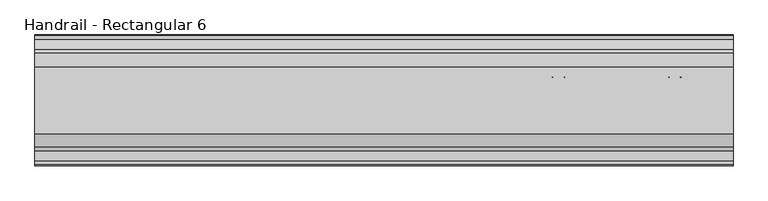
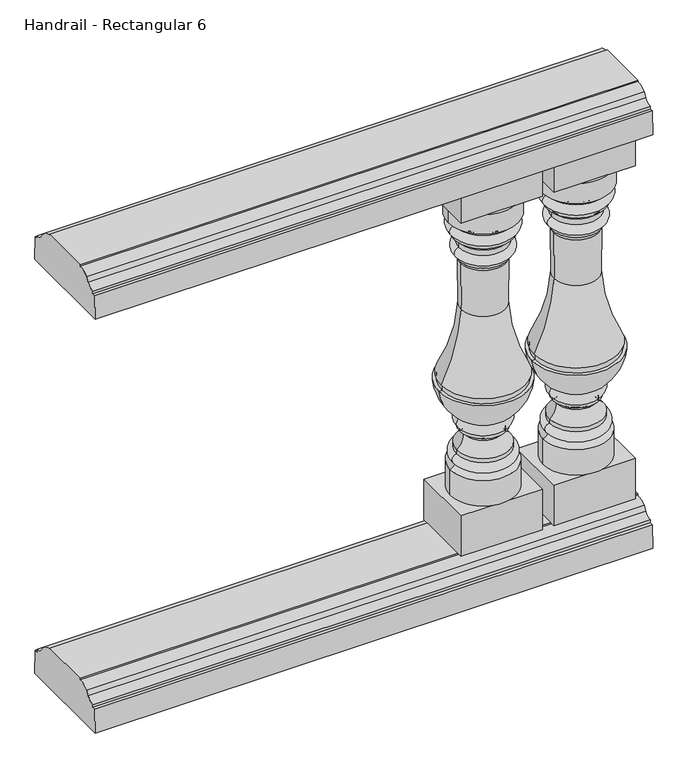
"""IFC4 building model written with IfcOpenShell, lengths in millimetres: railing geometry, Handrail - Rectangular 6."""

from ifc_helpers import new_model, si_unit, point, frame, frame_2d, origin, place, context, project, spatial, polyline, circle_curve, ellipse_curve, trimmed, segment, composite_curve, outline, extrude, source, transform, mapped, element, save
from ifc_brep_helpers import plane_surface, cylinder_surface, revolved_surface, advanced_brep


def handrail_rectangular_6_421e9862(model_context):
    return source(origin(), model_context, "Body", "SolidModel", [
        extrude(outline(composite_curve([segment(trimmed(circle_curve(frame_2d((-1771.1852268, 1054.89375)), 19.84375), [point((-1771.1852268, 1035.05))], [point((-1754.064785, 1044.8605607))], True, "CARTESIAN"), True, "CONTINUOUS"), segment(polyline([(-1754.064785, 1044.8605607), (-1747.604713, 1054.3201059)]), True, "CONTINUOUS"), segment(trimmed(circle_curve(frame_2d((-1723.5602268, 1027.90625)), 35.71875), [point((-1747.604713, 1054.3201059))], [point((-1723.5602268, 1063.625))], False, "CARTESIAN"), True, "CONTINUOUS"), segment(polyline([(-1723.5602268, 1063.625), (-1723.5602268, 1066.8), (-1607.6727268, 1066.8), (-1607.6727268, 1063.625)]), True, "CONTINUOUS"), segment(trimmed(circle_curve(frame_2d((-1607.6727268, 1027.90625)), 35.71875), [point((-1607.6727268, 1063.625))], [point((-1583.6282406, 1054.3201059))], False, "CARTESIAN"), True, "CONTINUOUS"), segment(polyline([(-1583.6282406, 1054.3201059), (-1577.1681686, 1044.8605607)]), True, "CONTINUOUS"), segment(trimmed(circle_curve(frame_2d((-1560.0477268, 1054.89375)), 19.84375), [point((-1577.1681686, 1044.8605607))], [point((-1560.0477268, 1035.05))], True, "CARTESIAN"), True, "CONTINUOUS"), segment(polyline([(-1560.0477268, 1035.05), (-1560.0477268, 1028.7), (-1552.9039768, 1028.7), (-1551.3164768, 974.725), (-1779.9164768, 974.725), (-1778.3289768, 1028.7), (-1771.1852268, 1028.7), (-1771.1852268, 1035.05)]), True, "CONTINUOUS")], self_intersect=False)), frame((18704.4521895, 0.0, 0.0), z_axis=(1.0, 0.0, 0.0), x_axis=(0.0, 1.0, 0.0)), (0.0, 0.0, 1.0), 1219.2),
        extrude(outline(composite_curve([segment(trimmed(circle_curve(frame_2d((-1771.1852268, 99.21875)), 19.84375), [point((-1771.1852268, 79.375))], [point((-1754.064785, 89.1855607))], True, "CARTESIAN"), True, "CONTINUOUS"), segment(polyline([(-1754.064785, 89.1855607), (-1747.604713, 98.6451059)]), True, "CONTINUOUS"), segment(trimmed(circle_curve(frame_2d((-1723.5602268, 72.23125)), 35.71875), [point((-1747.604713, 98.6451059))], [point((-1723.5602268, 107.95))], False, "CARTESIAN"), True, "CONTINUOUS"), segment(polyline([(-1723.5602268, 107.95), (-1723.5602268, 111.125), (-1607.6727268, 111.125), (-1607.6727268, 107.95)]), True, "CONTINUOUS"), segment(trimmed(circle_curve(frame_2d((-1607.6727268, 72.23125)), 35.71875), [point((-1607.6727268, 107.95))], [point((-1583.6282406, 98.6451059))], False, "CARTESIAN"), True, "CONTINUOUS"), segment(polyline([(-1583.6282406, 98.6451059), (-1577.1681686, 89.1855607)]), True, "CONTINUOUS"), segment(trimmed(circle_curve(frame_2d((-1560.0477268, 99.21875)), 19.84375), [point((-1577.1681686, 89.1855607))], [point((-1560.0477268, 79.375))], True, "CARTESIAN"), True, "CONTINUOUS"), segment(polyline([(-1560.0477268, 79.375), (-1560.0477268, 73.025), (-1552.9039768, 73.025), (-1551.3164768, 19.05), (-1779.9164768, 19.05), (-1778.3289768, 73.025), (-1771.1852268, 73.025), (-1771.1852268, 79.375)]), True, "CONTINUOUS")], self_intersect=False)), frame((18704.4521895, 0.0, 0.0), z_axis=(1.0, 0.0, 0.0), x_axis=(0.0, 1.0, 0.0)), (0.0, 0.0, 1.0), 1219.2),
        advanced_brep(
        [(19745.8521895, -1665.6164768, 881.0625), (19898.2521895, -1665.6164768, 881.0625), (19822.0521895, -1665.6164768, 881.0625), (19745.8521895, -1665.6164768, 835.3414358), (19898.2521895, -1665.6164768, 835.3414358), (19757.9812259, -1665.6164768, 824.1251909), (19886.1231531, -1665.6164768, 824.1251909), (19758.2264669, -1665.6164768, 801.0872354), (19885.8779121, -1665.6164768, 801.0872354), (19758.2264669, -1665.6164768, 792.9994382), (19885.8779121, -1665.6164768, 792.9994382), (19767.054986, -1665.6164768, 784.421477), (19877.049393, -1665.6164768, 784.421477), (19769.3912636, -1665.6164768, 770.116552), (19874.7131155, -1665.6164768, 770.116552), (19769.3912636, -1665.6164768, 748.0589375), (19874.7131155, -1665.6164768, 748.0589375), (19769.3912636, -1665.6164768, 739.775), (19874.7131155, -1665.6164768, 739.775), (19773.2635708, -1665.6164768, 732.0548389), (19870.8408083, -1665.6164768, 732.0548389), (19774.0730467, -1665.6164768, 625.8760562), (19870.0313324, -1665.6164768, 625.8760562), (19730.5137493, -1665.6164768, 465.93125), (19913.5906298, -1665.6164768, 465.93125), (19732.6156298, -1665.6164768, 465.93125), (19911.4887493, -1665.6164768, 465.93125), (19732.6156298, -1665.6164768, 453.23125), (19911.4887493, -1665.6164768, 453.23125), (19725.2146895, -1665.6164768, 453.23125), (19918.8896895, -1665.6164768, 453.23125), (19771.1407464, -1665.6164768, 375.8648455), (19872.9636327, -1665.6164768, 375.8648455), (19771.2821067, -1665.6164768, 352.5012686), (19872.8222724, -1665.6164768, 352.5012686), (19771.2821067, -1665.6164768, 345.021636), (19872.8222724, -1665.6164768, 345.021636), (19779.2341468, -1665.6164768, 336.1395712), (19864.8702323, -1665.6164768, 336.1395712), (19764.2656134, -1665.6164768, 304.3511281), (19879.8387657, -1665.6164768, 304.3511281), (19764.2656134, -1665.6164768, 295.0015923), (19879.8387657, -1665.6164768, 295.0015923), (19761.9267679, -1665.6164768, 273.4976463), (19882.1776112, -1665.6164768, 273.4976463), (19749.8419066, -1665.6164768, 263.7041906), (19894.2624725, -1665.6164768, 263.7041906), (19749.8419066, -1665.6164768, 204.7875), (19894.2624725, -1665.6164768, 204.7875), (19822.0521895, -1665.6164768, 204.7875)],
        [
            (0, 1, circle_curve(frame((19822.0521895, -1665.6164768, 881.0625), z_axis=(0.0, 0.0, 1.0), x_axis=(1.0, 0.0, 0.0)), 76.2)),
            (1, 2),
            (2, 0),
            (1, 0, circle_curve(frame((19822.0521895, -1665.6164768, 881.0625), z_axis=(0.0, 0.0, 1.0), x_axis=(1.0, 0.0, 0.0)), 76.2)),
            (3, 4, circle_curve(frame((19822.0521895, -1665.6164768, 835.3414358), z_axis=(0.0, 0.0, 1.0), x_axis=(1.0, 0.0, 0.0)), 76.2)),
            (4, 1),
            (0, 3),
            (4, 3, circle_curve(frame((19822.0521895, -1665.6164768, 835.3414358), z_axis=(0.0, 0.0, 1.0), x_axis=(1.0, 0.0, 0.0)), 76.2)),
            (5, 6, circle_curve(frame((19822.0521895, -1665.6164768, 824.1251909), z_axis=(0.0, 0.0, 1.0), x_axis=(1.0, 0.0, 0.0)), 64.0709636)),
            (6, 4, circle_curve(frame((19898.2657036, -1665.6164768, 823.1606434), z_axis=(0.0, 1.0, 0.0), x_axis=(-1.0, 0.0, 0.0)), 12.1807998)),
            (3, 5, circle_curve(frame((19745.8386755, -1665.6164768, 823.1606434), z_axis=(0.0, 1.0, 0.0), x_axis=(1.0, 0.0, 0.0)), 12.1807998)),
            (6, 5, circle_curve(frame((19822.0521895, -1665.6164768, 824.1251909), z_axis=(0.0, 0.0, 1.0), x_axis=(1.0, 0.0, 0.0)), 64.0709636)),
            (7, 8, circle_curve(frame((19822.0521895, -1665.6164768, 801.0872354), z_axis=(0.0, 0.0, 1.0), x_axis=(1.0, 0.0, 0.0)), 63.8257226)),
            (8, 6, circle_curve(frame((19883.7118198, -1665.6164768, 812.6305767), z_axis=(0.0, -1.0, 0.0), x_axis=(-1.0, 0.0, 0.0)), 11.7448152)),
            (5, 7, circle_curve(frame((19760.3925593, -1665.6164768, 812.6305767), z_axis=(0.0, -1.0, 0.0), x_axis=(1.0, 0.0, 0.0)), 11.7448152)),
            (8, 7, circle_curve(frame((19822.0521895, -1665.6164768, 801.0872354), z_axis=(0.0, 0.0, 1.0), x_axis=(1.0, 0.0, 0.0)), 63.8257226)),
            (9, 10, circle_curve(frame((19822.0521895, -1665.6164768, 792.9994382), z_axis=(0.0, 0.0, 1.0), x_axis=(1.0, 0.0, 0.0)), 63.8257226)),
            (10, 8),
            (7, 9),
            (10, 9, circle_curve(frame((19822.0521895, -1665.6164768, 792.9994382), z_axis=(0.0, 0.0, 1.0), x_axis=(1.0, 0.0, 0.0)), 63.8257226)),
            (11, 12, circle_curve(frame((19822.0521895, -1665.6164768, 784.421477), z_axis=(0.0, 0.0, 1.0), x_axis=(1.0, 0.0, 0.0)), 54.9972035)),
            (12, 10, circle_curve(frame((19890.2799215, -1665.6164768, 779.6366699), z_axis=(0.0, 1.0, 0.0), x_axis=(-1.0, 0.0, 0.0)), 14.06916)),
            (9, 11, circle_curve(frame((19753.8244576, -1665.6164768, 779.6366699), z_axis=(0.0, 1.0, 0.0), x_axis=(1.0, 0.0, 0.0)), 14.06916)),
            (12, 11, circle_curve(frame((19822.0521895, -1665.6164768, 784.421477), z_axis=(0.0, 0.0, 1.0), x_axis=(1.0, 0.0, 0.0)), 54.9972035)),
            (13, 14, circle_curve(frame((19822.0521895, -1665.6164768, 770.116552), z_axis=(0.0, 0.0, 1.0), x_axis=(1.0, 0.0, 0.0)), 52.660926)),
            (14, 12, circle_curve(frame((19903.672248, -1665.6164768, 772.7301948), z_axis=(0.0, 1.0, 0.0), x_axis=(-1.0, 0.0, 0.0)), 29.0768376)),
            (11, 13, circle_curve(frame((19740.4321311, -1665.6164768, 772.7301948), z_axis=(0.0, 1.0, 0.0), x_axis=(1.0, 0.0, 0.0)), 29.0768376)),
            (14, 13, circle_curve(frame((19822.0521895, -1665.6164768, 770.116552), z_axis=(0.0, 0.0, 1.0), x_axis=(1.0, 0.0, 0.0)), 52.660926)),
            (15, 16, circle_curve(frame((19822.0521895, -1665.6164768, 748.0589375), z_axis=(0.0, 0.0, 1.0), x_axis=(1.0, 0.0, 0.0)), 52.660926)),
            (16, 14, circle_curve(frame((19874.2588823, -1665.6164768, 759.0877448), z_axis=(0.0, -1.0, 0.0), x_axis=(-1.0, 0.0, 0.0)), 11.0381573)),
            (13, 15, circle_curve(frame((19769.8454968, -1665.6164768, 759.0877448), z_axis=(0.0, -1.0, 0.0), x_axis=(1.0, 0.0, 0.0)), 11.0381573)),
            (16, 15, circle_curve(frame((19822.0521895, -1665.6164768, 748.0589375), z_axis=(0.0, 0.0, 1.0), x_axis=(1.0, 0.0, 0.0)), 52.660926)),
            (17, 18, circle_curve(frame((19822.0521895, -1665.6164768, 739.775), z_axis=(0.0, 0.0, 1.0), x_axis=(1.0, 0.0, 0.0)), 52.660926)),
            (18, 16),
            (15, 17),
            (18, 17, circle_curve(frame((19822.0521895, -1665.6164768, 739.775), z_axis=(0.0, 0.0, 1.0), x_axis=(1.0, 0.0, 0.0)), 52.660926)),
            (19, 20, circle_curve(frame((19822.0521895, -1665.6164768, 732.0548389), z_axis=(0.0, 0.0, 1.0), x_axis=(1.0, 0.0, 0.0)), 48.7886187)),
            (20, 18, circle_curve(frame((19882.079759, -1665.6164768, 731.2487877), z_axis=(0.0, 1.0, 0.0), x_axis=(-1.0, 0.0, 0.0)), 11.2678184)),
            (17, 19, circle_curve(frame((19762.0246201, -1665.6164768, 731.2487877), z_axis=(0.0, 1.0, 0.0), x_axis=(1.0, 0.0, 0.0)), 11.2678184)),
            (20, 19, circle_curve(frame((19822.0521895, -1665.6164768, 732.0548389), z_axis=(0.0, 0.0, 1.0), x_axis=(1.0, 0.0, 0.0)), 48.7886187)),
            (21, 22, circle_curve(frame((19822.0521895, -1665.6164768, 625.8760562), z_axis=(0.0, 0.0, 1.0), x_axis=(1.0, 0.0, 0.0)), 47.9791428)),
            (22, 20, circle_curve(frame((20699.1718775, -1665.6164768, 672.6474087), z_axis=(0.0, 1.0, 0.0), x_axis=(-1.0, 0.0, 0.0)), 830.4586702)),
            (19, 21, circle_curve(frame((18944.9325016, -1665.6164768, 672.6474087), z_axis=(0.0, 1.0, 0.0), x_axis=(1.0, 0.0, 0.0)), 830.4586702)),
            (22, 21, circle_curve(frame((19822.0521895, -1665.6164768, 625.8760562), z_axis=(0.0, 0.0, 1.0), x_axis=(1.0, 0.0, 0.0)), 47.9791428)),
            (23, 24, circle_curve(frame((19822.0521895, -1665.6164768, 465.93125), z_axis=(0.0, 0.0, 1.0), x_axis=(1.0, 0.0, 0.0)), 91.5384403)),
            (24, 22, circle_curve(frame((20267.8631127, -1665.6164768, 648.3175235), z_axis=(0.0, 1.0, 0.0), x_axis=(-1.0, 0.0, 0.0)), 398.4642329)),
            (21, 23, circle_curve(frame((19376.2412664, -1665.6164768, 648.3175235), z_axis=(0.0, 1.0, 0.0), x_axis=(1.0, 0.0, 0.0)), 398.4642329)),
            (24, 23, circle_curve(frame((19822.0521895, -1665.6164768, 465.93125), z_axis=(0.0, 0.0, 1.0), x_axis=(1.0, 0.0, 0.0)), 91.5384403)),
            (25, 26, circle_curve(frame((19822.0521895, -1665.6164768, 465.93125), z_axis=(0.0, 0.0, 1.0), x_axis=(1.0, 0.0, 0.0)), 89.4365597)),
            (26, 24),
            (23, 25),
            (26, 25, circle_curve(frame((19822.0521895, -1665.6164768, 465.93125), z_axis=(0.0, 0.0, 1.0), x_axis=(1.0, 0.0, 0.0)), 89.4365597)),
            (27, 28, circle_curve(frame((19822.0521895, -1665.6164768, 453.23125), z_axis=(0.0, 0.0, 1.0), x_axis=(1.0, 0.0, 0.0)), 89.4365597)),
            (28, 26),
            (25, 27),
            (28, 27, circle_curve(frame((19822.0521895, -1665.6164768, 453.23125), z_axis=(0.0, 0.0, 1.0), x_axis=(1.0, 0.0, 0.0)), 89.4365597)),
            (29, 30, circle_curve(frame((19822.0521895, -1665.6164768, 453.23125), z_axis=(0.0, 0.0, 1.0), x_axis=(1.0, 0.0, 0.0)), 96.8375)),
            (30, 28),
            (27, 29),
            (30, 29, circle_curve(frame((19822.0521895, -1665.6164768, 453.23125), z_axis=(0.0, 0.0, 1.0), x_axis=(1.0, 0.0, 0.0)), 96.8375)),
            (31, 32, circle_curve(frame((19822.0521895, -1665.6164768, 375.8648455), z_axis=(0.0, 0.0, 1.0), x_axis=(1.0, 0.0, 0.0)), 50.9114432)),
            (32, 30, circle_curve(frame((19814.4105041, -1665.6164768, 462.9374706), z_axis=(0.0, -1.0, 0.0), x_axis=(-1.0, 0.0, 0.0)), 104.9290756)),
            (29, 31, circle_curve(frame((19829.6938749, -1665.6164768, 462.9374706), z_axis=(0.0, -1.0, 0.0), x_axis=(1.0, 0.0, 0.0)), 104.9290756)),
            (32, 31, circle_curve(frame((19822.0521895, -1665.6164768, 375.8648455), z_axis=(0.0, 0.0, 1.0), x_axis=(1.0, 0.0, 0.0)), 50.9114432)),
            (33, 34, circle_curve(frame((19822.0521895, -1665.6164768, 352.5012686), z_axis=(0.0, 0.0, 1.0), x_axis=(1.0, 0.0, 0.0)), 50.7700828)),
            (34, 32, circle_curve(frame((19867.5902787, -1665.6164768, 364.2151406), z_axis=(0.0, -1.0, 0.0), x_axis=(-1.0, 0.0, 0.0)), 12.8292072)),
            (31, 33, circle_curve(frame((19776.5141004, -1665.6164768, 364.2151406), z_axis=(0.0, -1.0, 0.0), x_axis=(1.0, 0.0, 0.0)), 12.8292072)),
            (34, 33, circle_curve(frame((19822.0521895, -1665.6164768, 352.5012686), z_axis=(0.0, 0.0, 1.0), x_axis=(1.0, 0.0, 0.0)), 50.7700828)),
            (35, 36, circle_curve(frame((19822.0521895, -1665.6164768, 345.021636), z_axis=(0.0, 0.0, 1.0), x_axis=(1.0, 0.0, 0.0)), 50.7700828)),
            (36, 34),
            (33, 35),
            (36, 35, circle_curve(frame((19822.0521895, -1665.6164768, 345.021636), z_axis=(0.0, 0.0, 1.0), x_axis=(1.0, 0.0, 0.0)), 50.7700828)),
            (37, 38, circle_curve(frame((19822.0521895, -1665.6164768, 336.1395712), z_axis=(0.0, 0.0, 1.0), x_axis=(1.0, 0.0, 0.0)), 42.8180427)),
            (38, 36, circle_curve(frame((19874.7676104, -1665.6164768, 335.27926), z_axis=(0.0, 1.0, 0.0), x_axis=(-1.0, 0.0, 0.0)), 9.9346983)),
            (35, 37, circle_curve(frame((19769.3367686, -1665.6164768, 335.27926), z_axis=(0.0, 1.0, 0.0), x_axis=(1.0, 0.0, 0.0)), 9.9346983)),
            (38, 37, circle_curve(frame((19822.0521895, -1665.6164768, 336.1395712), z_axis=(0.0, 0.0, 1.0), x_axis=(1.0, 0.0, 0.0)), 42.8180427)),
            (39, 40, circle_curve(frame((19822.0521895, -1665.6164768, 304.3511281), z_axis=(0.0, 0.0, 1.0), x_axis=(1.0, 0.0, 0.0)), 57.7865761)),
            (40, 38, circle_curve(frame((19899.6825509, -1665.6164768, 333.1135753), z_axis=(0.0, 1.0, 0.0), x_axis=(-1.0, 0.0, 0.0)), 34.9435857)),
            (37, 39, circle_curve(frame((19744.4218282, -1665.6164768, 333.1135753), z_axis=(0.0, 1.0, 0.0), x_axis=(1.0, 0.0, 0.0)), 34.9435857)),
            (40, 39, circle_curve(frame((19822.0521895, -1665.6164768, 304.3511281), z_axis=(0.0, 0.0, 1.0), x_axis=(1.0, 0.0, 0.0)), 57.7865761)),
            (41, 42, circle_curve(frame((19822.0521895, -1665.6164768, 295.0015923), z_axis=(0.0, 0.0, 1.0), x_axis=(1.0, 0.0, 0.0)), 57.7865761)),
            (42, 40),
            (39, 41),
            (42, 41, circle_curve(frame((19822.0521895, -1665.6164768, 295.0015923), z_axis=(0.0, 0.0, 1.0), x_axis=(1.0, 0.0, 0.0)), 57.7865761)),
            (43, 44, circle_curve(frame((19822.0521895, -1665.6164768, 273.4976463), z_axis=(0.0, 0.0, 1.0), x_axis=(1.0, 0.0, 0.0)), 60.1254216)),
            (44, 42, circle_curve(frame((19879.2247827, -1665.6164768, 284.0556497), z_axis=(0.0, -1.0, 0.0), x_axis=(-1.0, 0.0, 0.0)), 10.9631488)),
            (41, 43, circle_curve(frame((19764.8795963, -1665.6164768, 284.0556497), z_axis=(0.0, -1.0, 0.0), x_axis=(1.0, 0.0, 0.0)), 10.9631488)),
            (44, 43, circle_curve(frame((19822.0521895, -1665.6164768, 273.4976463), z_axis=(0.0, 0.0, 1.0), x_axis=(1.0, 0.0, 0.0)), 60.1254216)),
            (45, 46, circle_curve(frame((19822.0521895, -1665.6164768, 263.7041906), z_axis=(0.0, 0.0, 1.0), x_axis=(1.0, 0.0, 0.0)), 72.210283)),
            (46, 44, circle_curve(frame((19900.3933754, -1665.6164768, 283.622485), z_axis=(0.0, 1.0, 0.0), x_axis=(-1.0, 0.0, 0.0)), 20.8404996)),
            (43, 45, circle_curve(frame((19743.7110037, -1665.6164768, 283.622485), z_axis=(0.0, 1.0, 0.0), x_axis=(1.0, 0.0, 0.0)), 20.8404996)),
            (46, 45, circle_curve(frame((19822.0521895, -1665.6164768, 263.7041906), z_axis=(0.0, 0.0, 1.0), x_axis=(1.0, 0.0, 0.0)), 72.210283)),
            (47, 48, circle_curve(frame((19822.0521895, -1665.6164768, 204.7875), z_axis=(0.0, 0.0, 1.0), x_axis=(1.0, 0.0, 0.0)), 72.210283)),
            (48, 46),
            (45, 47),
            (48, 47, circle_curve(frame((19822.0521895, -1665.6164768, 204.7875), z_axis=(0.0, 0.0, 1.0), x_axis=(1.0, 0.0, 0.0)), 72.210283)),
            (49, 48),
            (47, 49),
        ],
        [
            plane_surface(frame((19822.0521895, -1665.6164768, 881.0625), z_axis=(0.0, 0.0, 1.0), x_axis=(1.0, 0.0, 0.0))),
            cylinder_surface(frame((19822.0521895, -1665.6164768, 833.4375), z_axis=(0.0, 0.0, -1.0), x_axis=(1.0, 0.0, 0.0)), 76.2),
            revolved_surface(trimmed(ellipse_curve(frame((19898.2657036, -1665.6164768, 823.1606434), z_axis=(0.0, -1.0, 0.0), x_axis=(-1.0, 0.0, 0.0)), 12.1807998, 12.1807998), [point((19898.2521895, -1665.6164768, 835.3414358))], [point((19886.1231531, -1665.6164768, 824.1251909))], True, "CARTESIAN"), (19822.0521895, -1665.6164768, 833.4375), (0.0, 0.0, -1.0)),
            revolved_surface(trimmed(ellipse_curve(frame((19883.7118198, -1665.6164768, 812.6305767), z_axis=(0.0, 1.0, 0.0), x_axis=(-1.0, 0.0, 0.0)), 11.7448152, 11.7448152), [point((19886.1231531, -1665.6164768, 824.1251909))], [point((19885.8779121, -1665.6164768, 801.0872354))], True, "CARTESIAN"), (19822.0521895, -1665.6164768, 833.4375), (0.0, 0.0, -1.0)),
            cylinder_surface(frame((19822.0521895, -1665.6164768, 833.4375), z_axis=(0.0, 0.0, -1.0), x_axis=(1.0, 0.0, 0.0)), 63.8257226),
            revolved_surface(trimmed(ellipse_curve(frame((19890.2799215, -1665.6164768, 779.6366699), z_axis=(0.0, -1.0, 0.0), x_axis=(-1.0, 0.0, 0.0)), 14.06916, 14.06916), [point((19885.8779121, -1665.6164768, 792.9994382))], [point((19877.049393, -1665.6164768, 784.421477))], True, "CARTESIAN"), (19822.0521895, -1665.6164768, 833.4375), (0.0, 0.0, -1.0)),
            revolved_surface(trimmed(ellipse_curve(frame((19903.672248, -1665.6164768, 772.7301948), z_axis=(0.0, -1.0, 0.0), x_axis=(-1.0, 0.0, 0.0)), 29.0768376, 29.0768376), [point((19877.049393, -1665.6164768, 784.421477))], [point((19874.7131155, -1665.6164768, 770.116552))], True, "CARTESIAN"), (19822.0521895, -1665.6164768, 833.4375), (0.0, 0.0, -1.0)),
            revolved_surface(trimmed(ellipse_curve(frame((19874.2588823, -1665.6164768, 759.0877448), z_axis=(0.0, 1.0, 0.0), x_axis=(-1.0, 0.0, 0.0)), 11.0381573, 11.0381573), [point((19874.7131155, -1665.6164768, 770.116552))], [point((19874.7131155, -1665.6164768, 748.0589375))], True, "CARTESIAN"), (19822.0521895, -1665.6164768, 833.4375), (0.0, 0.0, -1.0)),
            cylinder_surface(frame((19822.0521895, -1665.6164768, 833.4375), z_axis=(0.0, 0.0, -1.0), x_axis=(1.0, 0.0, 0.0)), 52.660926),
            revolved_surface(trimmed(ellipse_curve(frame((19882.079759, -1665.6164768, 731.2487877), z_axis=(0.0, -1.0, 0.0), x_axis=(-1.0, 0.0, 0.0)), 11.2678184, 11.2678184), [point((19874.7131155, -1665.6164768, 739.775))], [point((19870.8408083, -1665.6164768, 732.0548389))], True, "CARTESIAN"), (19822.0521895, -1665.6164768, 833.4375), (0.0, 0.0, -1.0)),
            revolved_surface(trimmed(ellipse_curve(frame((20699.1718775, -1665.6164768, 672.6474087), z_axis=(0.0, -1.0, 0.0), x_axis=(-1.0, 0.0, 0.0)), 830.4586702, 830.4586702), [point((19870.8408083, -1665.6164768, 732.0548389))], [point((19870.0313324, -1665.6164768, 625.8760562))], True, "CARTESIAN"), (19822.0521895, -1665.6164768, 833.4375), (0.0, 0.0, -1.0)),
            revolved_surface(trimmed(ellipse_curve(frame((20267.8631127, -1665.6164768, 648.3175235), z_axis=(0.0, -1.0, 0.0), x_axis=(-1.0, 0.0, 0.0)), 398.4642329, 398.4642329), [point((19870.0313324, -1665.6164768, 625.8760562))], [point((19913.5906298, -1665.6164768, 465.93125))], True, "CARTESIAN"), (19822.0521895, -1665.6164768, 833.4375), (0.0, 0.0, -1.0)),
            plane_surface(frame((19822.0521895, -1665.6164768, 465.93125), z_axis=(0.0, 0.0, -1.0), x_axis=(1.0, 0.0, 0.0))),
            cylinder_surface(frame((19822.0521895, -1665.6164768, 833.4375), z_axis=(0.0, 0.0, -1.0), x_axis=(1.0, 0.0, 0.0)), 89.4365597),
            plane_surface(frame((19822.0521895, -1665.6164768, 453.23125), z_axis=(0.0, 0.0, 1.0), x_axis=(1.0, 0.0, 0.0))),
            revolved_surface(trimmed(ellipse_curve(frame((19814.4105041, -1665.6164768, 462.9374706), z_axis=(0.0, 1.0, 0.0), x_axis=(-1.0, 0.0, 0.0)), 104.9290756, 104.9290756), [point((19918.8896895, -1665.6164768, 453.23125))], [point((19872.9636327, -1665.6164768, 375.8648455))], True, "CARTESIAN"), (19822.0521895, -1665.6164768, 833.4375), (0.0, 0.0, -1.0)),
            revolved_surface(trimmed(ellipse_curve(frame((19867.5902787, -1665.6164768, 364.2151406), z_axis=(0.0, 1.0, 0.0), x_axis=(-1.0, 0.0, 0.0)), 12.8292072, 12.8292072), [point((19872.9636327, -1665.6164768, 375.8648455))], [point((19872.8222724, -1665.6164768, 352.5012686))], True, "CARTESIAN"), (19822.0521895, -1665.6164768, 833.4375), (0.0, 0.0, -1.0)),
            cylinder_surface(frame((19822.0521895, -1665.6164768, 833.4375), z_axis=(0.0, 0.0, -1.0), x_axis=(1.0, 0.0, 0.0)), 50.7700828),
            revolved_surface(trimmed(ellipse_curve(frame((19874.7676104, -1665.6164768, 335.27926), z_axis=(0.0, -1.0, 0.0), x_axis=(-1.0, 0.0, 0.0)), 9.9346983, 9.9346983), [point((19872.8222724, -1665.6164768, 345.021636))], [point((19864.8702323, -1665.6164768, 336.1395712))], True, "CARTESIAN"), (19822.0521895, -1665.6164768, 833.4375), (0.0, 0.0, -1.0)),
            revolved_surface(trimmed(ellipse_curve(frame((19899.6825509, -1665.6164768, 333.1135753), z_axis=(0.0, -1.0, 0.0), x_axis=(-1.0, 0.0, 0.0)), 34.9435857, 34.9435857), [point((19864.8702323, -1665.6164768, 336.1395712))], [point((19879.8387657, -1665.6164768, 304.3511281))], True, "CARTESIAN"), (19822.0521895, -1665.6164768, 833.4375), (0.0, 0.0, -1.0)),
            cylinder_surface(frame((19822.0521895, -1665.6164768, 833.4375), z_axis=(0.0, 0.0, -1.0), x_axis=(1.0, 0.0, 0.0)), 57.7865761),
            revolved_surface(trimmed(ellipse_curve(frame((19879.2247827, -1665.6164768, 284.0556497), z_axis=(0.0, 1.0, 0.0), x_axis=(-1.0, 0.0, 0.0)), 10.9631488, 10.9631488), [point((19879.8387657, -1665.6164768, 295.0015923))], [point((19882.1776112, -1665.6164768, 273.4976463))], True, "CARTESIAN"), (19822.0521895, -1665.6164768, 833.4375), (0.0, 0.0, -1.0)),
            revolved_surface(trimmed(ellipse_curve(frame((19900.3933754, -1665.6164768, 283.622485), z_axis=(0.0, -1.0, 0.0), x_axis=(-1.0, 0.0, 0.0)), 20.8404996, 20.8404996), [point((19882.1776112, -1665.6164768, 273.4976463))], [point((19894.2624725, -1665.6164768, 263.7041906))], True, "CARTESIAN"), (19822.0521895, -1665.6164768, 833.4375), (0.0, 0.0, -1.0)),
            cylinder_surface(frame((19822.0521895, -1665.6164768, 833.4375), z_axis=(0.0, 0.0, -1.0), x_axis=(1.0, 0.0, 0.0)), 72.210283),
            plane_surface(frame((19822.0521895, -1665.6164768, 204.7875), z_axis=(0.0, 0.0, -1.0), x_axis=(1.0, 0.0, 0.0))),
        ],
        [
            (0, [[1, 2, 3]]),
            (0, [[4, -3, -2]]),
            (1, [[5, 6, -1, 7]]),
            (1, [[8, -7, -4, -6]]),
            (2, [[9, 10, -5, 11]]),
            (2, [[12, -11, -8, -10]]),
            (3, [[13, 14, -9, 15]]),
            (3, [[16, -15, -12, -14]]),
            (4, [[17, 18, -13, 19]]),
            (4, [[20, -19, -16, -18]]),
            (5, [[21, 22, -17, 23]]),
            (5, [[24, -23, -20, -22]]),
            (6, [[25, 26, -21, 27]]),
            (6, [[28, -27, -24, -26]]),
            (7, [[29, 30, -25, 31]]),
            (7, [[32, -31, -28, -30]]),
            (8, [[33, 34, -29, 35]]),
            (8, [[36, -35, -32, -34]]),
            (9, [[37, 38, -33, 39]]),
            (9, [[40, -39, -36, -38]]),
            (10, [[41, 42, -37, 43]]),
            (10, [[44, -43, -40, -42]]),
            (11, [[45, 46, -41, 47]]),
            (11, [[48, -47, -44, -46]]),
            (12, [[49, 50, -45, 51]]),
            (12, [[52, -51, -48, -50]]),
            (13, [[53, 54, -49, 55]]),
            (13, [[56, -55, -52, -54]]),
            (14, [[57, 58, -53, 59]]),
            (14, [[60, -59, -56, -58]]),
            (15, [[61, 62, -57, 63]]),
            (15, [[64, -63, -60, -62]]),
            (16, [[65, 66, -61, 67]]),
            (16, [[68, -67, -64, -66]]),
            (17, [[69, 70, -65, 71]]),
            (17, [[72, -71, -68, -70]]),
            (18, [[73, 74, -69, 75]]),
            (18, [[76, -75, -72, -74]]),
            (19, [[77, 78, -73, 79]]),
            (19, [[80, -79, -76, -78]]),
            (20, [[81, 82, -77, 83]]),
            (20, [[84, -83, -80, -82]]),
            (21, [[85, 86, -81, 87]]),
            (21, [[88, -87, -84, -86]]),
            (22, [[89, 90, -85, 91]]),
            (22, [[92, -91, -88, -90]]),
            (23, [[93, 94, -89, 95]]),
            (23, [[96, -95, -92, -94]]),
            (24, [[97, -93, 98]]),
            (24, [[-98, -96, -97]]),
        ],
    ),
        extrude(outline(polyline([(19733.1521895, -1735.4664768), (19733.1521895, -1595.7664768), (19910.9521895, -1595.7664768), (19910.9521895, -1735.4664768), (19733.1521895, -1735.4664768)])), frame((0.0, 0.0, 111.125), z_axis=(0.0, 0.0, 1.0), x_axis=(1.0, 0.0, 0.0)), (0.0, 0.0, 1.0), 93.6625),
        extrude(outline(polyline([(19733.1521895, -1595.7664768), (19910.9521895, -1595.7664768), (19910.9521895, -1735.4664768), (19733.1521895, -1735.4664768), (19733.1521895, -1595.7664768)])), frame((0.0, 0.0, 881.0625), z_axis=(0.0, 0.0, 1.0), x_axis=(1.0, 0.0, 0.0)), (0.0, 0.0, 1.0), 93.6625),
        advanced_brep(
        [(19542.6521895, -1665.6164768, 881.0625), (19695.0521895, -1665.6164768, 881.0625), (19618.8521895, -1665.6164768, 881.0625), (19542.6521895, -1665.6164768, 835.3414358), (19695.0521895, -1665.6164768, 835.3414358), (19554.7812259, -1665.6164768, 824.1251909), (19682.9231531, -1665.6164768, 824.1251909), (19555.0264669, -1665.6164768, 801.0872354), (19682.6779121, -1665.6164768, 801.0872354), (19555.0264669, -1665.6164768, 792.9994382), (19682.6779121, -1665.6164768, 792.9994382), (19563.854986, -1665.6164768, 784.421477), (19673.849393, -1665.6164768, 784.421477), (19566.1912636, -1665.6164768, 770.116552), (19671.5131155, -1665.6164768, 770.116552), (19566.1912636, -1665.6164768, 748.0589375), (19671.5131155, -1665.6164768, 748.0589375), (19566.1912636, -1665.6164768, 739.775), (19671.5131155, -1665.6164768, 739.775), (19570.0635708, -1665.6164768, 732.0548389), (19667.6408083, -1665.6164768, 732.0548389), (19570.8730467, -1665.6164768, 625.8760562), (19666.8313324, -1665.6164768, 625.8760562), (19527.3137493, -1665.6164768, 465.93125), (19710.3906298, -1665.6164768, 465.93125), (19529.4156298, -1665.6164768, 465.93125), (19708.2887493, -1665.6164768, 465.93125), (19529.4156298, -1665.6164768, 453.23125), (19708.2887493, -1665.6164768, 453.23125), (19522.0146895, -1665.6164768, 453.23125), (19715.6896895, -1665.6164768, 453.23125), (19567.9407464, -1665.6164768, 375.8648455), (19669.7636327, -1665.6164768, 375.8648455), (19568.0821067, -1665.6164768, 352.5012686), (19669.6222724, -1665.6164768, 352.5012686), (19568.0821067, -1665.6164768, 345.021636), (19669.6222724, -1665.6164768, 345.021636), (19576.0341468, -1665.6164768, 336.1395712), (19661.6702323, -1665.6164768, 336.1395712), (19561.0656134, -1665.6164768, 304.3511281), (19676.6387657, -1665.6164768, 304.3511281), (19561.0656134, -1665.6164768, 295.0015923), (19676.6387657, -1665.6164768, 295.0015923), (19558.7267679, -1665.6164768, 273.4976463), (19678.9776112, -1665.6164768, 273.4976463), (19546.6419066, -1665.6164768, 263.7041906), (19691.0624725, -1665.6164768, 263.7041906), (19546.6419066, -1665.6164768, 204.7875), (19691.0624725, -1665.6164768, 204.7875), (19618.8521895, -1665.6164768, 204.7875)],
        [
            (0, 1, circle_curve(frame((19618.8521895, -1665.6164768, 881.0625), z_axis=(0.0, 0.0, 1.0), x_axis=(1.0, 0.0, 0.0)), 76.2)),
            (1, 2),
            (2, 0),
            (1, 0, circle_curve(frame((19618.8521895, -1665.6164768, 881.0625), z_axis=(0.0, 0.0, 1.0), x_axis=(1.0, 0.0, 0.0)), 76.2)),
            (3, 4, circle_curve(frame((19618.8521895, -1665.6164768, 835.3414358), z_axis=(0.0, 0.0, 1.0), x_axis=(1.0, 0.0, 0.0)), 76.2)),
            (4, 1),
            (0, 3),
            (4, 3, circle_curve(frame((19618.8521895, -1665.6164768, 835.3414358), z_axis=(0.0, 0.0, 1.0), x_axis=(1.0, 0.0, 0.0)), 76.2)),
            (5, 6, circle_curve(frame((19618.8521895, -1665.6164768, 824.1251909), z_axis=(0.0, 0.0, 1.0), x_axis=(1.0, 0.0, 0.0)), 64.0709636)),
            (6, 4, circle_curve(frame((19695.0657036, -1665.6164768, 823.1606434), z_axis=(0.0, 1.0, 0.0), x_axis=(-1.0, 0.0, 0.0)), 12.1807998)),
            (3, 5, circle_curve(frame((19542.6386755, -1665.6164768, 823.1606434), z_axis=(0.0, 1.0, 0.0), x_axis=(1.0, 0.0, 0.0)), 12.1807998)),
            (6, 5, circle_curve(frame((19618.8521895, -1665.6164768, 824.1251909), z_axis=(0.0, 0.0, 1.0), x_axis=(1.0, 0.0, 0.0)), 64.0709636)),
            (7, 8, circle_curve(frame((19618.8521895, -1665.6164768, 801.0872354), z_axis=(0.0, 0.0, 1.0), x_axis=(1.0, 0.0, 0.0)), 63.8257226)),
            (8, 6, circle_curve(frame((19680.5118198, -1665.6164768, 812.6305767), z_axis=(0.0, -1.0, 0.0), x_axis=(-1.0, 0.0, 0.0)), 11.7448152)),
            (5, 7, circle_curve(frame((19557.1925593, -1665.6164768, 812.6305767), z_axis=(0.0, -1.0, 0.0), x_axis=(1.0, 0.0, 0.0)), 11.7448152)),
            (8, 7, circle_curve(frame((19618.8521895, -1665.6164768, 801.0872354), z_axis=(0.0, 0.0, 1.0), x_axis=(1.0, 0.0, 0.0)), 63.8257226)),
            (9, 10, circle_curve(frame((19618.8521895, -1665.6164768, 792.9994382), z_axis=(0.0, 0.0, 1.0), x_axis=(1.0, 0.0, 0.0)), 63.8257226)),
            (10, 8),
            (7, 9),
            (10, 9, circle_curve(frame((19618.8521895, -1665.6164768, 792.9994382), z_axis=(0.0, 0.0, 1.0), x_axis=(1.0, 0.0, 0.0)), 63.8257226)),
            (11, 12, circle_curve(frame((19618.8521895, -1665.6164768, 784.421477), z_axis=(0.0, 0.0, 1.0), x_axis=(1.0, 0.0, 0.0)), 54.9972035)),
            (12, 10, circle_curve(frame((19687.0799215, -1665.6164768, 779.6366699), z_axis=(0.0, 1.0, 0.0), x_axis=(-1.0, 0.0, 0.0)), 14.06916)),
            (9, 11, circle_curve(frame((19550.6244576, -1665.6164768, 779.6366699), z_axis=(0.0, 1.0, 0.0), x_axis=(1.0, 0.0, 0.0)), 14.06916)),
            (12, 11, circle_curve(frame((19618.8521895, -1665.6164768, 784.421477), z_axis=(0.0, 0.0, 1.0), x_axis=(1.0, 0.0, 0.0)), 54.9972035)),
            (13, 14, circle_curve(frame((19618.8521895, -1665.6164768, 770.116552), z_axis=(0.0, 0.0, 1.0), x_axis=(1.0, 0.0, 0.0)), 52.660926)),
            (14, 12, circle_curve(frame((19700.472248, -1665.6164768, 772.7301948), z_axis=(0.0, 1.0, 0.0), x_axis=(-1.0, 0.0, 0.0)), 29.0768376)),
            (11, 13, circle_curve(frame((19537.2321311, -1665.6164768, 772.7301948), z_axis=(0.0, 1.0, 0.0), x_axis=(1.0, 0.0, 0.0)), 29.0768376)),
            (14, 13, circle_curve(frame((19618.8521895, -1665.6164768, 770.116552), z_axis=(0.0, 0.0, 1.0), x_axis=(1.0, 0.0, 0.0)), 52.660926)),
            (15, 16, circle_curve(frame((19618.8521895, -1665.6164768, 748.0589375), z_axis=(0.0, 0.0, 1.0), x_axis=(1.0, 0.0, 0.0)), 52.660926)),
            (16, 14, circle_curve(frame((19671.0588823, -1665.6164768, 759.0877448), z_axis=(0.0, -1.0, 0.0), x_axis=(-1.0, 0.0, 0.0)), 11.0381573)),
            (13, 15, circle_curve(frame((19566.6454968, -1665.6164768, 759.0877448), z_axis=(0.0, -1.0, 0.0), x_axis=(1.0, 0.0, 0.0)), 11.0381573)),
            (16, 15, circle_curve(frame((19618.8521895, -1665.6164768, 748.0589375), z_axis=(0.0, 0.0, 1.0), x_axis=(1.0, 0.0, 0.0)), 52.660926)),
            (17, 18, circle_curve(frame((19618.8521895, -1665.6164768, 739.775), z_axis=(0.0, 0.0, 1.0), x_axis=(1.0, 0.0, 0.0)), 52.660926)),
            (18, 16),
            (15, 17),
            (18, 17, circle_curve(frame((19618.8521895, -1665.6164768, 739.775), z_axis=(0.0, 0.0, 1.0), x_axis=(1.0, 0.0, 0.0)), 52.660926)),
            (19, 20, circle_curve(frame((19618.8521895, -1665.6164768, 732.0548389), z_axis=(0.0, 0.0, 1.0), x_axis=(1.0, 0.0, 0.0)), 48.7886187)),
            (20, 18, circle_curve(frame((19678.879759, -1665.6164768, 731.2487877), z_axis=(0.0, 1.0, 0.0), x_axis=(-1.0, 0.0, 0.0)), 11.2678184)),
            (17, 19, circle_curve(frame((19558.8246201, -1665.6164768, 731.2487877), z_axis=(0.0, 1.0, 0.0), x_axis=(1.0, 0.0, 0.0)), 11.2678184)),
            (20, 19, circle_curve(frame((19618.8521895, -1665.6164768, 732.0548389), z_axis=(0.0, 0.0, 1.0), x_axis=(1.0, 0.0, 0.0)), 48.7886187)),
            (21, 22, circle_curve(frame((19618.8521895, -1665.6164768, 625.8760562), z_axis=(0.0, 0.0, 1.0), x_axis=(1.0, 0.0, 0.0)), 47.9791428)),
            (22, 20, circle_curve(frame((20495.9718775, -1665.6164768, 672.6474087), z_axis=(0.0, 1.0, 0.0), x_axis=(-1.0, 0.0, 0.0)), 830.4586702)),
            (19, 21, circle_curve(frame((18741.7325016, -1665.6164768, 672.6474087), z_axis=(0.0, 1.0, 0.0), x_axis=(1.0, 0.0, 0.0)), 830.4586702)),
            (22, 21, circle_curve(frame((19618.8521895, -1665.6164768, 625.8760562), z_axis=(0.0, 0.0, 1.0), x_axis=(1.0, 0.0, 0.0)), 47.9791428)),
            (23, 24, circle_curve(frame((19618.8521895, -1665.6164768, 465.93125), z_axis=(0.0, 0.0, 1.0), x_axis=(1.0, 0.0, 0.0)), 91.5384403)),
            (24, 22, circle_curve(frame((20064.6631127, -1665.6164768, 648.3175235), z_axis=(0.0, 1.0, 0.0), x_axis=(-1.0, 0.0, 0.0)), 398.4642329)),
            (21, 23, circle_curve(frame((19173.0412664, -1665.6164768, 648.3175235), z_axis=(0.0, 1.0, 0.0), x_axis=(1.0, 0.0, 0.0)), 398.4642329)),
            (24, 23, circle_curve(frame((19618.8521895, -1665.6164768, 465.93125), z_axis=(0.0, 0.0, 1.0), x_axis=(1.0, 0.0, 0.0)), 91.5384403)),
            (25, 26, circle_curve(frame((19618.8521895, -1665.6164768, 465.93125), z_axis=(0.0, 0.0, 1.0), x_axis=(1.0, 0.0, 0.0)), 89.4365597)),
            (26, 24),
            (23, 25),
            (26, 25, circle_curve(frame((19618.8521895, -1665.6164768, 465.93125), z_axis=(0.0, 0.0, 1.0), x_axis=(1.0, 0.0, 0.0)), 89.4365597)),
            (27, 28, circle_curve(frame((19618.8521895, -1665.6164768, 453.23125), z_axis=(0.0, 0.0, 1.0), x_axis=(1.0, 0.0, 0.0)), 89.4365597)),
            (28, 26),
            (25, 27),
            (28, 27, circle_curve(frame((19618.8521895, -1665.6164768, 453.23125), z_axis=(0.0, 0.0, 1.0), x_axis=(1.0, 0.0, 0.0)), 89.4365597)),
            (29, 30, circle_curve(frame((19618.8521895, -1665.6164768, 453.23125), z_axis=(0.0, 0.0, 1.0), x_axis=(1.0, 0.0, 0.0)), 96.8375)),
            (30, 28),
            (27, 29),
            (30, 29, circle_curve(frame((19618.8521895, -1665.6164768, 453.23125), z_axis=(0.0, 0.0, 1.0), x_axis=(1.0, 0.0, 0.0)), 96.8375)),
            (31, 32, circle_curve(frame((19618.8521895, -1665.6164768, 375.8648455), z_axis=(0.0, 0.0, 1.0), x_axis=(1.0, 0.0, 0.0)), 50.9114432)),
            (32, 30, circle_curve(frame((19611.2105041, -1665.6164768, 462.9374706), z_axis=(0.0, -1.0, 0.0), x_axis=(-1.0, 0.0, 0.0)), 104.9290756)),
            (29, 31, circle_curve(frame((19626.4938749, -1665.6164768, 462.9374706), z_axis=(0.0, -1.0, 0.0), x_axis=(1.0, 0.0, 0.0)), 104.9290756)),
            (32, 31, circle_curve(frame((19618.8521895, -1665.6164768, 375.8648455), z_axis=(0.0, 0.0, 1.0), x_axis=(1.0, 0.0, 0.0)), 50.9114432)),
            (33, 34, circle_curve(frame((19618.8521895, -1665.6164768, 352.5012686), z_axis=(0.0, 0.0, 1.0), x_axis=(1.0, 0.0, 0.0)), 50.7700828)),
            (34, 32, circle_curve(frame((19664.3902787, -1665.6164768, 364.2151406), z_axis=(0.0, -1.0, 0.0), x_axis=(-1.0, 0.0, 0.0)), 12.8292072)),
            (31, 33, circle_curve(frame((19573.3141004, -1665.6164768, 364.2151406), z_axis=(0.0, -1.0, 0.0), x_axis=(1.0, 0.0, 0.0)), 12.8292072)),
            (34, 33, circle_curve(frame((19618.8521895, -1665.6164768, 352.5012686), z_axis=(0.0, 0.0, 1.0), x_axis=(1.0, 0.0, 0.0)), 50.7700828)),
            (35, 36, circle_curve(frame((19618.8521895, -1665.6164768, 345.021636), z_axis=(0.0, 0.0, 1.0), x_axis=(1.0, 0.0, 0.0)), 50.7700828)),
            (36, 34),
            (33, 35),
            (36, 35, circle_curve(frame((19618.8521895, -1665.6164768, 345.021636), z_axis=(0.0, 0.0, 1.0), x_axis=(1.0, 0.0, 0.0)), 50.7700828)),
            (37, 38, circle_curve(frame((19618.8521895, -1665.6164768, 336.1395712), z_axis=(0.0, 0.0, 1.0), x_axis=(1.0, 0.0, 0.0)), 42.8180427)),
            (38, 36, circle_curve(frame((19671.5676104, -1665.6164768, 335.27926), z_axis=(0.0, 1.0, 0.0), x_axis=(-1.0, 0.0, 0.0)), 9.9346983)),
            (35, 37, circle_curve(frame((19566.1367686, -1665.6164768, 335.27926), z_axis=(0.0, 1.0, 0.0), x_axis=(1.0, 0.0, 0.0)), 9.9346983)),
            (38, 37, circle_curve(frame((19618.8521895, -1665.6164768, 336.1395712), z_axis=(0.0, 0.0, 1.0), x_axis=(1.0, 0.0, 0.0)), 42.8180427)),
            (39, 40, circle_curve(frame((19618.8521895, -1665.6164768, 304.3511281), z_axis=(0.0, 0.0, 1.0), x_axis=(1.0, 0.0, 0.0)), 57.7865761)),
            (40, 38, circle_curve(frame((19696.4825509, -1665.6164768, 333.1135753), z_axis=(0.0, 1.0, 0.0), x_axis=(-1.0, 0.0, 0.0)), 34.9435857)),
            (37, 39, circle_curve(frame((19541.2218282, -1665.6164768, 333.1135753), z_axis=(0.0, 1.0, 0.0), x_axis=(1.0, 0.0, 0.0)), 34.9435857)),
            (40, 39, circle_curve(frame((19618.8521895, -1665.6164768, 304.3511281), z_axis=(0.0, 0.0, 1.0), x_axis=(1.0, 0.0, 0.0)), 57.7865761)),
            (41, 42, circle_curve(frame((19618.8521895, -1665.6164768, 295.0015923), z_axis=(0.0, 0.0, 1.0), x_axis=(1.0, 0.0, 0.0)), 57.7865761)),
            (42, 40),
            (39, 41),
            (42, 41, circle_curve(frame((19618.8521895, -1665.6164768, 295.0015923), z_axis=(0.0, 0.0, 1.0), x_axis=(1.0, 0.0, 0.0)), 57.7865761)),
            (43, 44, circle_curve(frame((19618.8521895, -1665.6164768, 273.4976463), z_axis=(0.0, 0.0, 1.0), x_axis=(1.0, 0.0, 0.0)), 60.1254216)),
            (44, 42, circle_curve(frame((19676.0247827, -1665.6164768, 284.0556497), z_axis=(0.0, -1.0, 0.0), x_axis=(-1.0, 0.0, 0.0)), 10.9631488)),
            (41, 43, circle_curve(frame((19561.6795963, -1665.6164768, 284.0556497), z_axis=(0.0, -1.0, 0.0), x_axis=(1.0, 0.0, 0.0)), 10.9631488)),
            (44, 43, circle_curve(frame((19618.8521895, -1665.6164768, 273.4976463), z_axis=(0.0, 0.0, 1.0), x_axis=(1.0, 0.0, 0.0)), 60.1254216)),
            (45, 46, circle_curve(frame((19618.8521895, -1665.6164768, 263.7041906), z_axis=(0.0, 0.0, 1.0), x_axis=(1.0, 0.0, 0.0)), 72.210283)),
            (46, 44, circle_curve(frame((19697.1933754, -1665.6164768, 283.622485), z_axis=(0.0, 1.0, 0.0), x_axis=(-1.0, 0.0, 0.0)), 20.8404996)),
            (43, 45, circle_curve(frame((19540.5110037, -1665.6164768, 283.622485), z_axis=(0.0, 1.0, 0.0), x_axis=(1.0, 0.0, 0.0)), 20.8404996)),
            (46, 45, circle_curve(frame((19618.8521895, -1665.6164768, 263.7041906), z_axis=(0.0, 0.0, 1.0), x_axis=(1.0, 0.0, 0.0)), 72.210283)),
            (47, 48, circle_curve(frame((19618.8521895, -1665.6164768, 204.7875), z_axis=(0.0, 0.0, 1.0), x_axis=(1.0, 0.0, 0.0)), 72.210283)),
            (48, 46),
            (45, 47),
            (48, 47, circle_curve(frame((19618.8521895, -1665.6164768, 204.7875), z_axis=(0.0, 0.0, 1.0), x_axis=(1.0, 0.0, 0.0)), 72.210283)),
            (49, 48),
            (47, 49),
        ],
        [
            plane_surface(frame((19618.8521895, -1665.6164768, 881.0625), z_axis=(0.0, 0.0, 1.0), x_axis=(1.0, 0.0, 0.0))),
            cylinder_surface(frame((19618.8521895, -1665.6164768, 833.4375), z_axis=(0.0, 0.0, -1.0), x_axis=(1.0, 0.0, 0.0)), 76.2),
            revolved_surface(trimmed(ellipse_curve(frame((19695.0657036, -1665.6164768, 823.1606434), z_axis=(0.0, -1.0, 0.0), x_axis=(-1.0, 0.0, 0.0)), 12.1807998, 12.1807998), [point((19695.0521895, -1665.6164768, 835.3414358))], [point((19682.9231531, -1665.6164768, 824.1251909))], True, "CARTESIAN"), (19618.8521895, -1665.6164768, 833.4375), (0.0, 0.0, -1.0)),
            revolved_surface(trimmed(ellipse_curve(frame((19680.5118198, -1665.6164768, 812.6305767), z_axis=(0.0, 1.0, 0.0), x_axis=(-1.0, 0.0, 0.0)), 11.7448152, 11.7448152), [point((19682.9231531, -1665.6164768, 824.1251909))], [point((19682.6779121, -1665.6164768, 801.0872354))], True, "CARTESIAN"), (19618.8521895, -1665.6164768, 833.4375), (0.0, 0.0, -1.0)),
            cylinder_surface(frame((19618.8521895, -1665.6164768, 833.4375), z_axis=(0.0, 0.0, -1.0), x_axis=(1.0, 0.0, 0.0)), 63.8257226),
            revolved_surface(trimmed(ellipse_curve(frame((19687.0799215, -1665.6164768, 779.6366699), z_axis=(0.0, -1.0, 0.0), x_axis=(-1.0, 0.0, 0.0)), 14.06916, 14.06916), [point((19682.6779121, -1665.6164768, 792.9994382))], [point((19673.849393, -1665.6164768, 784.421477))], True, "CARTESIAN"), (19618.8521895, -1665.6164768, 833.4375), (0.0, 0.0, -1.0)),
            revolved_surface(trimmed(ellipse_curve(frame((19700.472248, -1665.6164768, 772.7301948), z_axis=(0.0, -1.0, 0.0), x_axis=(-1.0, 0.0, 0.0)), 29.0768376, 29.0768376), [point((19673.849393, -1665.6164768, 784.421477))], [point((19671.5131155, -1665.6164768, 770.116552))], True, "CARTESIAN"), (19618.8521895, -1665.6164768, 833.4375), (0.0, 0.0, -1.0)),
            revolved_surface(trimmed(ellipse_curve(frame((19671.0588823, -1665.6164768, 759.0877448), z_axis=(0.0, 1.0, 0.0), x_axis=(-1.0, 0.0, 0.0)), 11.0381573, 11.0381573), [point((19671.5131155, -1665.6164768, 770.116552))], [point((19671.5131155, -1665.6164768, 748.0589375))], True, "CARTESIAN"), (19618.8521895, -1665.6164768, 833.4375), (0.0, 0.0, -1.0)),
            cylinder_surface(frame((19618.8521895, -1665.6164768, 833.4375), z_axis=(0.0, 0.0, -1.0), x_axis=(1.0, 0.0, 0.0)), 52.660926),
            revolved_surface(trimmed(ellipse_curve(frame((19678.879759, -1665.6164768, 731.2487877), z_axis=(0.0, -1.0, 0.0), x_axis=(-1.0, 0.0, 0.0)), 11.2678184, 11.2678184), [point((19671.5131155, -1665.6164768, 739.775))], [point((19667.6408083, -1665.6164768, 732.0548389))], True, "CARTESIAN"), (19618.8521895, -1665.6164768, 833.4375), (0.0, 0.0, -1.0)),
            revolved_surface(trimmed(ellipse_curve(frame((20495.9718775, -1665.6164768, 672.6474087), z_axis=(0.0, -1.0, 0.0), x_axis=(-1.0, 0.0, 0.0)), 830.4586702, 830.4586702), [point((19667.6408083, -1665.6164768, 732.0548389))], [point((19666.8313324, -1665.6164768, 625.8760562))], True, "CARTESIAN"), (19618.8521895, -1665.6164768, 833.4375), (0.0, 0.0, -1.0)),
            revolved_surface(trimmed(ellipse_curve(frame((20064.6631127, -1665.6164768, 648.3175235), z_axis=(0.0, -1.0, 0.0), x_axis=(-1.0, 0.0, 0.0)), 398.4642329, 398.4642329), [point((19666.8313324, -1665.6164768, 625.8760562))], [point((19710.3906298, -1665.6164768, 465.93125))], True, "CARTESIAN"), (19618.8521895, -1665.6164768, 833.4375), (0.0, 0.0, -1.0)),
            plane_surface(frame((19618.8521895, -1665.6164768, 465.93125), z_axis=(0.0, 0.0, -1.0), x_axis=(1.0, 0.0, 0.0))),
            cylinder_surface(frame((19618.8521895, -1665.6164768, 833.4375), z_axis=(0.0, 0.0, -1.0), x_axis=(1.0, 0.0, 0.0)), 89.4365597),
            plane_surface(frame((19618.8521895, -1665.6164768, 453.23125), z_axis=(0.0, 0.0, 1.0), x_axis=(1.0, 0.0, 0.0))),
            revolved_surface(trimmed(ellipse_curve(frame((19611.2105041, -1665.6164768, 462.9374706), z_axis=(0.0, 1.0, 0.0), x_axis=(-1.0, 0.0, 0.0)), 104.9290756, 104.9290756), [point((19715.6896895, -1665.6164768, 453.23125))], [point((19669.7636327, -1665.6164768, 375.8648455))], True, "CARTESIAN"), (19618.8521895, -1665.6164768, 833.4375), (0.0, 0.0, -1.0)),
            revolved_surface(trimmed(ellipse_curve(frame((19664.3902787, -1665.6164768, 364.2151406), z_axis=(0.0, 1.0, 0.0), x_axis=(-1.0, 0.0, 0.0)), 12.8292072, 12.8292072), [point((19669.7636327, -1665.6164768, 375.8648455))], [point((19669.6222724, -1665.6164768, 352.5012686))], True, "CARTESIAN"), (19618.8521895, -1665.6164768, 833.4375), (0.0, 0.0, -1.0)),
            cylinder_surface(frame((19618.8521895, -1665.6164768, 833.4375), z_axis=(0.0, 0.0, -1.0), x_axis=(1.0, 0.0, 0.0)), 50.7700828),
            revolved_surface(trimmed(ellipse_curve(frame((19671.5676104, -1665.6164768, 335.27926), z_axis=(0.0, -1.0, 0.0), x_axis=(-1.0, 0.0, 0.0)), 9.9346983, 9.9346983), [point((19669.6222724, -1665.6164768, 345.021636))], [point((19661.6702323, -1665.6164768, 336.1395712))], True, "CARTESIAN"), (19618.8521895, -1665.6164768, 833.4375), (0.0, 0.0, -1.0)),
            revolved_surface(trimmed(ellipse_curve(frame((19696.4825509, -1665.6164768, 333.1135753), z_axis=(0.0, -1.0, 0.0), x_axis=(-1.0, 0.0, 0.0)), 34.9435857, 34.9435857), [point((19661.6702323, -1665.6164768, 336.1395712))], [point((19676.6387657, -1665.6164768, 304.3511281))], True, "CARTESIAN"), (19618.8521895, -1665.6164768, 833.4375), (0.0, 0.0, -1.0)),
            cylinder_surface(frame((19618.8521895, -1665.6164768, 833.4375), z_axis=(0.0, 0.0, -1.0), x_axis=(1.0, 0.0, 0.0)), 57.7865761),
            revolved_surface(trimmed(ellipse_curve(frame((19676.0247827, -1665.6164768, 284.0556497), z_axis=(0.0, 1.0, 0.0), x_axis=(-1.0, 0.0, 0.0)), 10.9631488, 10.9631488), [point((19676.6387657, -1665.6164768, 295.0015923))], [point((19678.9776112, -1665.6164768, 273.4976463))], True, "CARTESIAN"), (19618.8521895, -1665.6164768, 833.4375), (0.0, 0.0, -1.0)),
            revolved_surface(trimmed(ellipse_curve(frame((19697.1933754, -1665.6164768, 283.622485), z_axis=(0.0, -1.0, 0.0), x_axis=(-1.0, 0.0, 0.0)), 20.8404996, 20.8404996), [point((19678.9776112, -1665.6164768, 273.4976463))], [point((19691.0624725, -1665.6164768, 263.7041906))], True, "CARTESIAN"), (19618.8521895, -1665.6164768, 833.4375), (0.0, 0.0, -1.0)),
            cylinder_surface(frame((19618.8521895, -1665.6164768, 833.4375), z_axis=(0.0, 0.0, -1.0), x_axis=(1.0, 0.0, 0.0)), 72.210283),
            plane_surface(frame((19618.8521895, -1665.6164768, 204.7875), z_axis=(0.0, 0.0, -1.0), x_axis=(1.0, 0.0, 0.0))),
        ],
        [
            (0, [[1, 2, 3]]),
            (0, [[4, -3, -2]]),
            (1, [[5, 6, -1, 7]]),
            (1, [[8, -7, -4, -6]]),
            (2, [[9, 10, -5, 11]]),
            (2, [[12, -11, -8, -10]]),
            (3, [[13, 14, -9, 15]]),
            (3, [[16, -15, -12, -14]]),
            (4, [[17, 18, -13, 19]]),
            (4, [[20, -19, -16, -18]]),
            (5, [[21, 22, -17, 23]]),
            (5, [[24, -23, -20, -22]]),
            (6, [[25, 26, -21, 27]]),
            (6, [[28, -27, -24, -26]]),
            (7, [[29, 30, -25, 31]]),
            (7, [[32, -31, -28, -30]]),
            (8, [[33, 34, -29, 35]]),
            (8, [[36, -35, -32, -34]]),
            (9, [[37, 38, -33, 39]]),
            (9, [[40, -39, -36, -38]]),
            (10, [[41, 42, -37, 43]]),
            (10, [[44, -43, -40, -42]]),
            (11, [[45, 46, -41, 47]]),
            (11, [[48, -47, -44, -46]]),
            (12, [[49, 50, -45, 51]]),
            (12, [[52, -51, -48, -50]]),
            (13, [[53, 54, -49, 55]]),
            (13, [[56, -55, -52, -54]]),
            (14, [[57, 58, -53, 59]]),
            (14, [[60, -59, -56, -58]]),
            (15, [[61, 62, -57, 63]]),
            (15, [[64, -63, -60, -62]]),
            (16, [[65, 66, -61, 67]]),
            (16, [[68, -67, -64, -66]]),
            (17, [[69, 70, -65, 71]]),
            (17, [[72, -71, -68, -70]]),
            (18, [[73, 74, -69, 75]]),
            (18, [[76, -75, -72, -74]]),
            (19, [[77, 78, -73, 79]]),
            (19, [[80, -79, -76, -78]]),
            (20, [[81, 82, -77, 83]]),
            (20, [[84, -83, -80, -82]]),
            (21, [[85, 86, -81, 87]]),
            (21, [[88, -87, -84, -86]]),
            (22, [[89, 90, -85, 91]]),
            (22, [[92, -91, -88, -90]]),
            (23, [[93, 94, -89, 95]]),
            (23, [[96, -95, -92, -94]]),
            (24, [[97, -93, 98]]),
            (24, [[-98, -96, -97]]),
        ],
    ),
        extrude(outline(polyline([(19529.9521895, -1735.4664768), (19529.9521895, -1595.7664768), (19707.7521895, -1595.7664768), (19707.7521895, -1735.4664768), (19529.9521895, -1735.4664768)])), frame((0.0, 0.0, 111.125), z_axis=(0.0, 0.0, 1.0), x_axis=(1.0, 0.0, 0.0)), (0.0, 0.0, 1.0), 93.6625),
        extrude(outline(polyline([(19529.9521895, -1595.7664768), (19707.7521895, -1595.7664768), (19707.7521895, -1735.4664768), (19529.9521895, -1735.4664768), (19529.9521895, -1595.7664768)])), frame((0.0, 0.0, 881.0625), z_axis=(0.0, 0.0, 1.0), x_axis=(1.0, 0.0, 0.0)), (0.0, 0.0, 1.0), 93.6625),
    ])


if __name__ == "__main__":
    model = new_model("IFC4")
    model_context = context("Model", 3, world=origin())
    ifc_project = project(units=[si_unit("LENGTHUNIT", "METRE", prefix="MILLI")], contexts=[model_context])
    site = spatial("IfcSite", under=ifc_project)
    building = spatial("IfcBuilding", under=site)
    placement = place(None, origin())
    handrail_rectangular_6_shape = handrail_rectangular_6_421e9862(model_context)
    element("IfcRailing", 1, ObjectType="Handrail - Rectangular 6", at=placement, inside=building, context=model_context, shape_type="MappedRepresentation", body=[
        mapped(handrail_rectangular_6_shape, transform((0.0, 0.0, 0.0), x_axis=(1.0, 0.0, 0.0), y_axis=(0.0, 1.0, 0.0), z_axis=(0.0, 0.0, 1.0))),
    ])
    save(model, "model.ifc")
